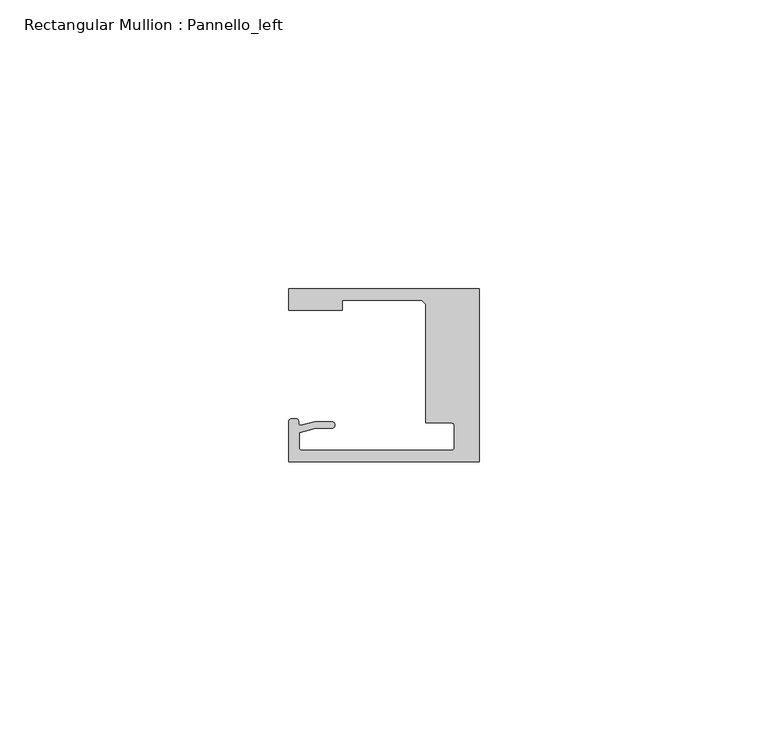
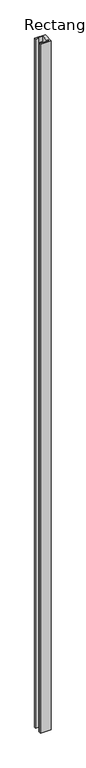
"""IFC4 building model written with IfcOpenShell, lengths in millimetres: member geometry, Rectangular Mullion : Pannello_left."""

from ifc_helpers import new_model, si_unit, frame, origin, place, context, project, spatial, polyline, circle_curve, source, transform, mapped, element, save
from ifc_brep_helpers import plane_surface, cylinder_surface, revolved_surface, extruded_surface, spline_curve, advanced_brep


def rectangular_mullion_pannello_left_9f49ba5d(model_context):
    return source(origin(), model_context, "Body", "AdvancedBrep", [
        advanced_brep(
        [(-33.0, 15.0, 0.0), (-33.0, 11.3000004, 0.0), (-23.700041, 11.3000004, 0.0), (-23.700041, 13.0000004, 0.0), (-10.0000103, 13.0000004, 0.0), (-9.2999726, 12.2999849, 0.0), (-9.2999726, -8.2500595, 0.0), (-4.7999726, -8.2500595, 0.0), (-4.2999726, -8.7500595, 0.0), (-4.2999726, -12.50001, 0.0), (-4.7999726, -13.00001, 0.0), (-30.69998, -13.00001, 0.0), (-31.19998, -12.50001, 0.0), (-31.19998, -9.9657591, 0.0), (-28.3419477, -9.1999523, 0.0), (-25.59998, -9.1999523, 0.0), (-25.59998, -7.9999523, 0.0), (-28.4999305, -7.9999523, 0.0), (-30.9223017, -8.6490241, 0.0), (-33.0000135, -8.0000472, 0.0), (-33.0000135, -15.0, 0.0), (0.0, -15.0, 0.0), (0.0, 15.0, 0.0), (-33.0, 15.0, -2240.0), (0.0, 15.0, -2240.0), (0.0, -15.0, -2240.0), (-33.0000135, -15.0, -2240.0), (-33.0000135, -8.0000472, -2240.0), (-30.9223017, -8.6490241, -2240.0), (-28.4999305, -7.9999523, -2240.0), (-25.59998, -7.9999523, -2240.0), (-25.59998, -9.1999523, -2240.0), (-28.3419477, -9.1999523, -2240.0), (-31.19998, -9.9657591, -2240.0), (-31.19998, -12.50001, -2240.0), (-30.69998, -13.00001, -2240.0), (-4.7999726, -13.00001, -2240.0), (-4.2999726, -12.50001, -2240.0), (-4.2999726, -8.7500595, -2240.0), (-4.7999726, -8.2500595, -2240.0), (-9.2999726, -8.2500595, -2240.0), (-9.2999726, 12.2999849, -2240.0), (-10.0000103, 13.0000004, -2240.0), (-23.700041, 13.0000004, -2240.0), (-23.700041, 11.3000004, -2240.0), (-33.0, 11.3000004, -2240.0)],
        [
            (0, 1),
            (1, 2),
            (2, 3),
            (3, 4),
            (4, 5),
            (5, 6),
            (6, 7),
            (7, 8, circle_curve(frame((-4.7999726, -8.7500595, 0.0), z_axis=(0.0, 0.0, -1.0), x_axis=(0.0, 1.0, 0.0)), 0.5)),
            (8, 9),
            (9, 10, circle_curve(frame((-4.7999726, -12.50001, 0.0), z_axis=(0.0, 0.0, -1.0), x_axis=(1.0, 0.0, 0.0)), 0.5)),
            (10, 11),
            (11, 12, circle_curve(frame((-30.69998, -12.50001, 0.0), z_axis=(0.0, 0.0, -1.0), x_axis=(0.0, -1.0, 0.0)), 0.5)),
            (12, 13),
            (13, 14),
            (14, 15),
            (15, 16, circle_curve(frame((-25.59998, -8.5999523, 0.0), z_axis=(0.0, 0.0, 1.0), x_axis=(0.0, -1.0, 0.0)), 0.6)),
            (16, 17),
            (17, 18),
            (18, 19, spline_curve(3, [(-30.9223017, -8.6490241, 0.0), (-31.312054066, -8.717747958, 0.0), (-31.298563602, -8.366228555, 0.0), (-31.305645054, -7.690065204, 0.0), (-31.357433266, -7.563996614, 0.0), (-32.262327879, -7.456527435, 0.0), (-33.0000135, -7.457047519, 0.0), (-33.0000135, -8.0000472, 0.0)], [4, 2, 2, 4], [0.0, 0.001840817752199412, 0.004996616814974408, 0.007702013405570312])),
            (19, 20),
            (20, 21),
            (21, 22),
            (22, 0),
            (23, 24),
            (24, 25),
            (25, 26),
            (26, 27),
            (27, 28, spline_curve(3, [(-33.0000135, -8.0000472, -2240.0), (-33.0000135, -7.457047519, -2240.0), (-32.262327879, -7.456527435, -2240.0), (-31.357433266, -7.563996614, -2240.0), (-31.305645054, -7.690065204, -2240.0), (-31.298563602, -8.366228555, -2240.0), (-31.312054066, -8.717747958, -2240.0), (-30.9223017, -8.6490241, -2240.0)], [4, 2, 2, 4], [0.0, 0.0027053965905959043, 0.0058611956533709, 0.007702013405570312])),
            (28, 29),
            (29, 30),
            (30, 31, circle_curve(frame((-25.59998, -8.5999523, -2240.0), z_axis=(0.0, 0.0, -1.0), x_axis=(0.0, -1.0, 0.0)), 0.6)),
            (31, 32),
            (32, 33),
            (33, 34),
            (34, 35, circle_curve(frame((-30.69998, -12.50001, -2240.0), z_axis=(0.0, 0.0, 1.0), x_axis=(0.0, -1.0, 0.0)), 0.5)),
            (35, 36),
            (36, 37, circle_curve(frame((-4.7999726, -12.50001, -2240.0), z_axis=(0.0, 0.0, 1.0), x_axis=(1.0, 0.0, 0.0)), 0.5)),
            (37, 38),
            (38, 39, circle_curve(frame((-4.7999726, -8.7500595, -2240.0), z_axis=(0.0, 0.0, 1.0), x_axis=(0.0, 1.0, 0.0)), 0.5)),
            (39, 40),
            (40, 41),
            (41, 42),
            (42, 43),
            (43, 44),
            (44, 45),
            (45, 23),
            (0, 23),
            (45, 1),
            (44, 2),
            (43, 3),
            (42, 4),
            (41, 5),
            (40, 6),
            (39, 7),
            (38, 8),
            (37, 9),
            (36, 10),
            (35, 11),
            (34, 12),
            (33, 13),
            (32, 14),
            (31, 15),
            (30, 16),
            (29, 17),
            (28, 18),
            (27, 19),
            (26, 20),
            (25, 21),
            (24, 22),
        ],
        [
            plane_surface(frame((0.0, -36.2491502, 0.0), z_axis=(0.0, 0.0, 1.0), x_axis=(-1.0, 0.0, 0.0))),
            plane_surface(frame((0.0, -36.2491502, -2240.0), z_axis=(0.0, 0.0, -1.0), x_axis=(-1.0, 0.0, 0.0))),
            plane_surface(frame((-33.0, 15.0, 0.0), z_axis=(-1.0, 0.0, 0.0), x_axis=(0.0, 0.0, -1.0))),
            plane_surface(frame((-33.0, 11.3000004, 0.0), z_axis=(0.0, -1.0, 0.0), x_axis=(0.0, 0.0, -1.0))),
            plane_surface(frame((-23.700041, 11.3000004, 0.0), z_axis=(1.0, 0.0, 0.0), x_axis=(0.0, 0.0, -1.0))),
            plane_surface(frame((-23.700041, 13.0000004, 0.0), z_axis=(0.0, -1.0, 0.0), x_axis=(0.0, 0.0, -1.0))),
            plane_surface(frame((-10.0000103, 13.0000004, 0.0), z_axis=(-0.7070955486277984, -0.7071180135668678, 0.0), x_axis=(0.0, 0.0, -1.0))),
            plane_surface(frame((-9.2999726, 12.2999849, 0.0), z_axis=(-1.0, 0.0, 0.0), x_axis=(0.0, 0.0, -1.0))),
            plane_surface(frame((-9.2999726, -8.2500595, 0.0), z_axis=(0.0, -1.0, 0.0), x_axis=(0.0, 0.0, -1.0))),
            revolved_surface(polyline([(-4.7999726, -8.2500595, -2240.0), (-4.7999726, -8.2500595, 0.0)]), (-4.7999726, -8.7500595, 0.0), (0.0, 0.0, -1.0)),
            plane_surface(frame((-4.2999726, -8.7500595, 0.0), z_axis=(-1.0, 0.0, 0.0), x_axis=(0.0, 0.0, -1.0))),
            revolved_surface(polyline([(-4.2999726, -12.50001, -2240.0), (-4.2999726, -12.50001, 0.0)]), (-4.7999726, -12.50001, 0.0), (0.0, 0.0, -1.0)),
            plane_surface(frame((-4.7999726, -13.00001, 0.0), z_axis=(0.0, 1.0, 0.0), x_axis=(0.0, 0.0, -1.0))),
            revolved_surface(polyline([(-30.69998, -13.00001, -2240.0), (-30.69998, -13.00001, 0.0)]), (-30.69998, -12.50001, 0.0), (0.0, 0.0, -1.0)),
            plane_surface(frame((-31.19998, -12.50001, 0.0), z_axis=(1.0, 0.0, 0.0), x_axis=(0.0, 0.0, -1.0))),
            plane_surface(frame((-31.19998, -9.9657591, 0.0), z_axis=(0.25881883204288636, -0.9659258833782002, 0.0), x_axis=(0.0, 0.0, -1.0))),
            plane_surface(frame((-28.3419477, -9.1999523, 0.0), z_axis=(0.0, -1.0, 0.0), x_axis=(0.0, 0.0, -1.0))),
            cylinder_surface(frame((-25.59998, -8.5999523, 0.0), z_axis=(0.0, 0.0, 1.0), x_axis=(0.0, -1.0, 0.0)), 0.6),
            plane_surface(frame((-25.59998, -7.9999523, 0.0), z_axis=(0.0, 1.0, 0.0), x_axis=(0.0, 0.0, -1.0))),
            plane_surface(frame((-28.4999305, -7.9999523, 0.0), z_axis=(-0.25881883200192934, 0.9659258833891746, 0.0), x_axis=(0.0, 0.0, -1.0))),
            extruded_surface(spline_curve(3, [(-30.9223017, -8.6490241, -2240.0), (-31.312054066, -8.717747958, -2240.0), (-31.298563602, -8.366228555, -2240.0), (-31.305645054, -7.690065204, -2240.0), (-31.357433266, -7.563996614, -2240.0), (-32.262327879, -7.456527435, -2240.0), (-33.0000135, -7.457047519, -2240.0), (-33.0000135, -8.0000472, -2240.0)], [4, 2, 2, 4], [0.0, 0.001840817752199412, 0.004996616814974408, 0.007702013405570312]), (0.0, 0.0, 2240.0), 2240.0),
            plane_surface(frame((-33.0000135, -8.0000472, 0.0), z_axis=(-1.0, 0.0, 0.0), x_axis=(0.0, 0.0, -1.0))),
            plane_surface(frame((-33.0000135, -15.0, 0.0), z_axis=(0.0, -1.0, 0.0), x_axis=(0.0, 0.0, -1.0))),
            plane_surface(frame((0.0, -15.0, 0.0), z_axis=(1.0, 0.0, 0.0), x_axis=(0.0, 0.0, -1.0))),
            plane_surface(frame((0.0, 15.0, 0.0), z_axis=(0.0, 1.0, 0.0), x_axis=(0.0, 0.0, -1.0))),
        ],
        [
            (0, [[1, 2, 3, 4, 5, 6, 7, 8, 9, 10, 11, 12, 13, 14, 15, 16, 17, 18, 19, 20, 21, 22, 23]]),
            (1, [[24, 25, 26, 27, 28, 29, 30, 31, 32, 33, 34, 35, 36, 37, 38, 39, 40, 41, 42, 43, 44, 45, 46]]),
            (2, [[-1, 47, -46, 48]]),
            (3, [[-2, -48, -45, 49]]),
            (4, [[-3, -49, -44, 50]]),
            (5, [[-4, -50, -43, 51]]),
            (6, [[-5, -51, -42, 52]]),
            (7, [[-6, -52, -41, 53]]),
            (8, [[-7, -53, -40, 54]]),
            (9, [[-8, -54, -39, 55]]),
            (10, [[-9, -55, -38, 56]]),
            (11, [[-10, -56, -37, 57]]),
            (12, [[-11, -57, -36, 58]]),
            (13, [[-12, -58, -35, 59]]),
            (14, [[-13, -59, -34, 60]]),
            (15, [[-14, -60, -33, 61]]),
            (16, [[-15, -61, -32, 62]]),
            (17, [[-16, -62, -31, 63]]),
            (18, [[-17, -63, -30, 64]]),
            (19, [[-18, -64, -29, 65]]),
            (20, [[-19, -65, -28, 66]]),
            (21, [[-20, -66, -27, 67]]),
            (22, [[-21, -67, -26, 68]]),
            (23, [[-22, -68, -25, 69]]),
            (24, [[-23, -69, -24, -47]]),
        ],
    ),
    ])


if __name__ == "__main__":
    model = new_model("IFC4")
    model_context = context("Model", 3, world=origin())
    ifc_project = project(units=[si_unit("LENGTHUNIT", "METRE", prefix="MILLI")], contexts=[model_context])
    site = spatial("IfcSite", under=ifc_project)
    building = spatial("IfcBuilding", under=site)
    placement = place(None, origin())
    rectangular_mullion_pannello_left_shape = rectangular_mullion_pannello_left_9f49ba5d(model_context)
    element("IfcMember", 1, ObjectType="Rectangular Mullion : Pannello_left", at=placement, inside=building, context=model_context, shape_type="MappedRepresentation", body=[
        mapped(rectangular_mullion_pannello_left_shape, transform((0.0, 0.0, 0.0), x_axis=(1.0, 0.0, 0.0), y_axis=(0.0, 1.0, 0.0), z_axis=(0.0, 0.0, 1.0))),
    ])
    save(model, "model.ifc")

# Revit data of these elements
# Type "Rectangular Mullion : Pannello_left"
#   built-in parameter 1007322 = 0.0984252 (stored number, unit not read)
#   built-in parameter 1007320 = 0.0305117 (stored number, unit not read)
